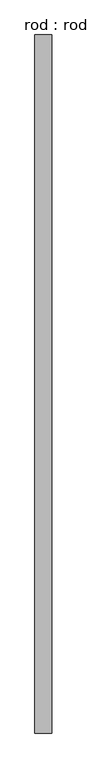
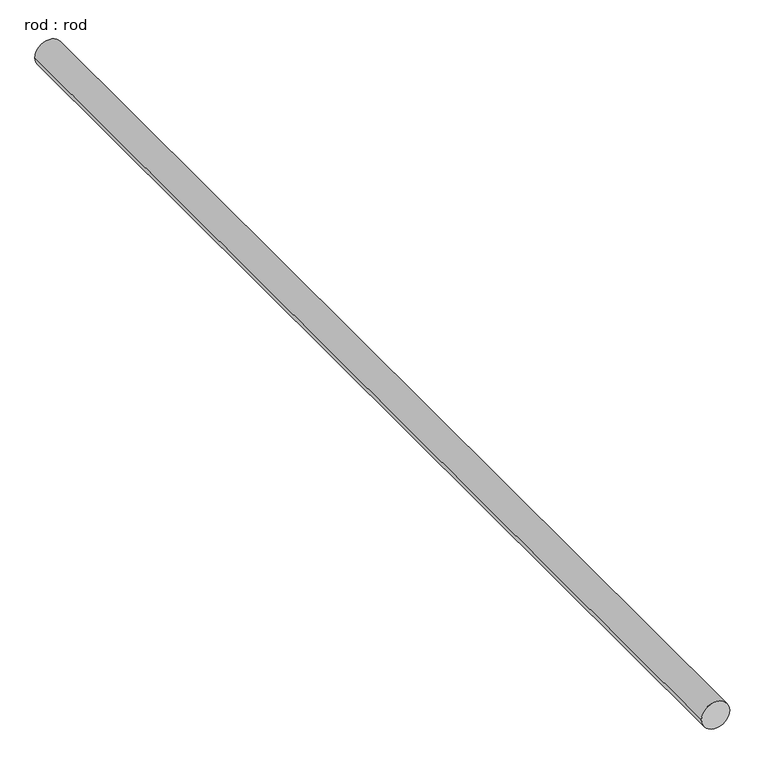
"""IFC4 building model written with IfcOpenShell, lengths in millimetres: proxy geometry, rod : rod."""

from ifc_helpers import new_model, si_unit, point, frame, frame_2d, origin, place, context, project, spatial, circle_curve, trimmed, segment, composite_curve, outline, extrude, source, transform, mapped, element, save


def rod_rod_ae7010cc(model_context):
    return source(origin(), model_context, "Body", "SweptSolid", [
        extrude(outline(composite_curve([segment(trimmed(circle_curve(frame_2d((0.0108462, 0.0)), 200.0), [point((0.0108462, 200.0))], [point((0.0108462, -200.0))], False, "CARTESIAN"), True, "CONTINUOUS"), segment(trimmed(circle_curve(frame_2d((0.0108462, 0.0)), 200.0), [point((0.0108462, -200.0))], [point((0.0108462, 200.0))], False, "CARTESIAN"), True, "CONTINUOUS")], self_intersect=False)), frame((0.0, -4090.4385714, 0.0), z_axis=(0.0, 1.0, 0.0), x_axis=(0.0, 0.0, 1.0)), (0.0, 0.0, 1.0), 16366.3343735),
    ])


if __name__ == "__main__":
    model = new_model("IFC4")
    model_context = context("Model", 3, world=origin())
    ifc_project = project(units=[si_unit("LENGTHUNIT", "METRE", prefix="MILLI")], contexts=[model_context])
    site = spatial("IfcSite", under=ifc_project)
    building = spatial("IfcBuilding", under=site)
    placement = place(None, origin())
    rod_rod_shape = rod_rod_ae7010cc(model_context)
    element("IfcBuildingElementProxy", 1, Name="rod : rod", ObjectType="rod : rod", at=placement, inside=building, context=model_context, shape_type="MappedRepresentation", body=[
        mapped(rod_rod_shape, transform((0.0, 0.0, 0.0), x_axis=(1.0, 0.0, 0.0), y_axis=(0.0, 1.0, 0.0), z_axis=(0.0, 0.0, 1.0))),
    ])
    save(model, "model.ifc")

# Revit data of these elements
# Type "rod : rod"
#   Default Elevation = 0
